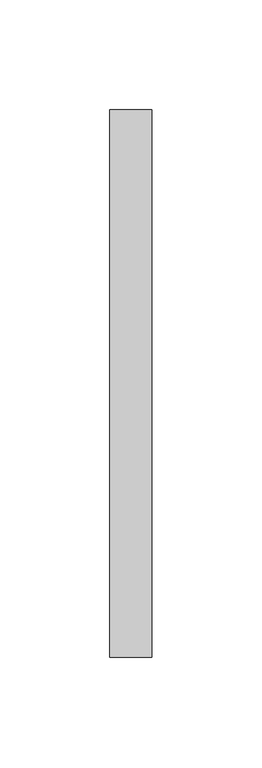
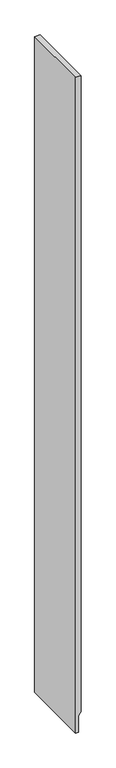
"""IFC4 building model written with IfcOpenShell, lengths in millimetres: proxy geometry, Generic Models 7:Generic Models 1:5:Generic Models 1:5 : Generic Models 7:Generic Models 1:337419:22 : Generic Models 7:Generic Models 1:5:Generic Models 1:5 : Generic Models 7:Generic Models 1:337419:311462."""

from ifc_helpers import new_model, si_unit, frame, origin, place, context, project, spatial, polyline, outline, extrude, source, transform, mapped, element, save


def generic_models_9f9e0187(model_context):
    return source(origin(), model_context, "Body", "SweptSolid", [
        extrude(outline(polyline([(3723.834699, 560337.2810188), (3784.758103, 560337.2810188), (3795.8780043, 560346.6117239), (6155.090949, 560346.6117239), (6155.090949, 560327.5617239), (3723.834699, 560327.5617239), (3723.834699, 560337.2810188)])), frame((0.0, -579000.6913841, 0.0), z_axis=(0.0, 1.0, 0.0), x_axis=(0.0, 0.0, 1.0)), (0.0, 0.0, 1.0), 249.0712362),
    ])


if __name__ == "__main__":
    model = new_model("IFC4")
    model_context = context("Model", 3, world=origin())
    ifc_project = project(units=[si_unit("LENGTHUNIT", "METRE", prefix="MILLI")], contexts=[model_context])
    site = spatial("IfcSite", under=ifc_project)
    building = spatial("IfcBuilding", under=site)
    placement = place(None, origin())
    generic_models_shape = generic_models_9f9e0187(model_context)
    element("IfcBuildingElementProxy", 1, Name="Generic Models 7:Generic Models 1:5:Generic Models 1:5 : Generic Models 7:Generic Models 1:337419:22 : Generic Models 7:Generic Models 1:5:Generic Models 1:5 : Generic Models 7:Generic Models 1:337419:311462", ObjectType="Generic Models 7:Generic Models 1:5:Generic Models 1:5 : Generic Models 7:Generic Models 1:337419:22 : Generic Models 7:Generic Models 1:5:Generic Models 1:5 : Generic Models 7:Generic Models 1:337419:311462", at=placement, inside=building, context=model_context, shape_type="MappedRepresentation", body=[
        mapped(generic_models_shape, transform((0.0, 0.0, 0.0), x_axis=(1.0, 0.0, 0.0), y_axis=(0.0, 1.0, 0.0), z_axis=(0.0, 0.0, 1.0))),
    ])
    save(model, "model.ifc")

# Revit data of these elements
# Type "Generic Models 7:Generic Models 1:5:Generic Models 1:5 : Generic Models 7:Generic Models 1:337419:22 : Generic Models 7:Generic Models 1:5:Generic Models 1:5 : Generic Models 7:Generic Models 1:337419:311462"
#   NameOverride = "Generic Models 7:Generic Models 1:5:Generic Models 1:5 : Generic Models 7:Generic Models 1:337419:311462"
#   ObjectTypeOverride = "Generic Models 1:5 : Generic Models 7:Generic Models 1:337419"
#   Reference = "Generic Models 1"
#   Tag = "311462"
# Element 1 (IfcBuildingElementProxy, "Generic Models 7:Generic Models 1:5:Generic Models 1:5 : Generic Models 7:Generic Models 1:337419:22 : Generic Models 7:Generic Models 1:5:Generic Models 1:5 : Generic Models 7:Generic Models 1:337419:311462")
#   Materials on its faces: "1\" MINERAL WOOL BOARD INSULATION"
# Materials
#   "1\" MINERAL WOOL BOARD INSULATION": class "Unassigned", colour RGB 205 188 106, transparency 0, Cost = 0
